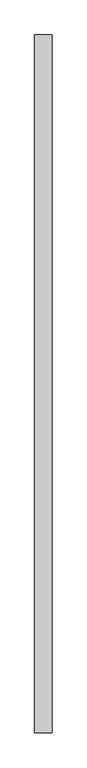
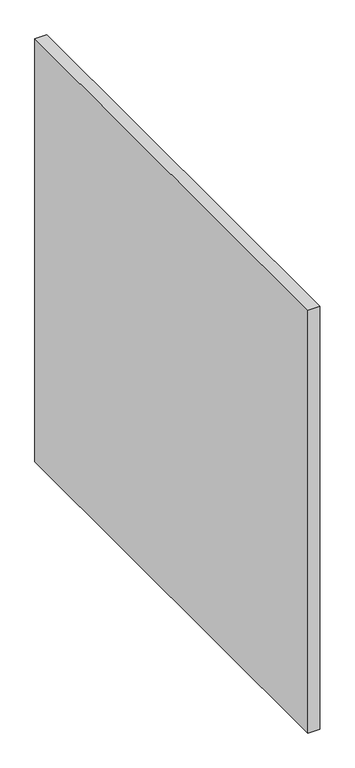
"""IFC4 building model written with IfcOpenShell, lengths in millimetres: proxy geometry, Generic Models 7:Generic Models 1:5:Generic Models 1:5 : Generic Models 7:Generic Models 1:337419:27 : Generic Models 7:Generic Models 1:5:Generic Models 1:5 : Generic Models 7:Generic Models 1:337419:311462."""

from ifc_helpers import new_model, si_unit, frame, origin, place, context, project, spatial, polyline, outline, extrude, source, transform, mapped, element, save


def generic_models_cf09a48e(model_context):
    return source(origin(), model_context, "Body", "SweptSolid", [
        extrude(outline(polyline([(578901.3117239, -568215.2163841), (578647.3117239, -568215.2163841), (578647.3117239, -558080.616384), (578901.3117239, -558080.616384), (578901.3117239, -568215.2163841)])), frame((0.0, 0.0, -158.1372439), z_axis=(0.0, 0.0, 1.0), x_axis=(1.0, 0.0, 0.0)), (0.0, 0.0, 1.0), 9585.4979353),
    ])


if __name__ == "__main__":
    model = new_model("IFC4")
    model_context = context("Model", 3, world=origin())
    ifc_project = project(units=[si_unit("LENGTHUNIT", "METRE", prefix="MILLI")], contexts=[model_context])
    site = spatial("IfcSite", under=ifc_project)
    building = spatial("IfcBuilding", under=site)
    placement = place(None, origin())
    generic_models_shape = generic_models_cf09a48e(model_context)
    element("IfcBuildingElementProxy", 1, Name="Generic Models 7:Generic Models 1:5:Generic Models 1:5 : Generic Models 7:Generic Models 1:337419:27 : Generic Models 7:Generic Models 1:5:Generic Models 1:5 : Generic Models 7:Generic Models 1:337419:311462", ObjectType="Generic Models 7:Generic Models 1:5:Generic Models 1:5 : Generic Models 7:Generic Models 1:337419:27 : Generic Models 7:Generic Models 1:5:Generic Models 1:5 : Generic Models 7:Generic Models 1:337419:311462", at=placement, inside=building, context=model_context, shape_type="MappedRepresentation", body=[
        mapped(generic_models_shape, transform((0.0, 0.0, 0.0), x_axis=(1.0, 0.0, 0.0), y_axis=(0.0, 1.0, 0.0), z_axis=(0.0, 0.0, 1.0))),
    ])
    save(model, "model.ifc")

# Revit data of these elements
# Type "Generic Models 7:Generic Models 1:5:Generic Models 1:5 : Generic Models 7:Generic Models 1:337419:27 : Generic Models 7:Generic Models 1:5:Generic Models 1:5 : Generic Models 7:Generic Models 1:337419:311462"
#   NameOverride = "Generic Models 7:Generic Models 1:5:Generic Models 1:5 : Generic Models 7:Generic Models 1:337419:311462"
#   ObjectTypeOverride = "Generic Models 1:5 : Generic Models 7:Generic Models 1:337419"
#   Reference = "Generic Models 1"
#   Tag = "311462"
# Element 1 (IfcBuildingElementProxy, "Generic Models 7:Generic Models 1:5:Generic Models 1:5 : Generic Models 7:Generic Models 1:337419:27 : Generic Models 7:Generic Models 1:5:Generic Models 1:5 : Generic Models 7:Generic Models 1:337419:311462")
#   Materials on its faces: "SIMPLE SAVER INSULATION WITH LINER - COLOR: WHITE"
# Materials
#   "SIMPLE SAVER INSULATION WITH LINER - COLOR: WHITE": class "Unassigned", colour RGB 219 193 225, transparency 0, Cost = 0
